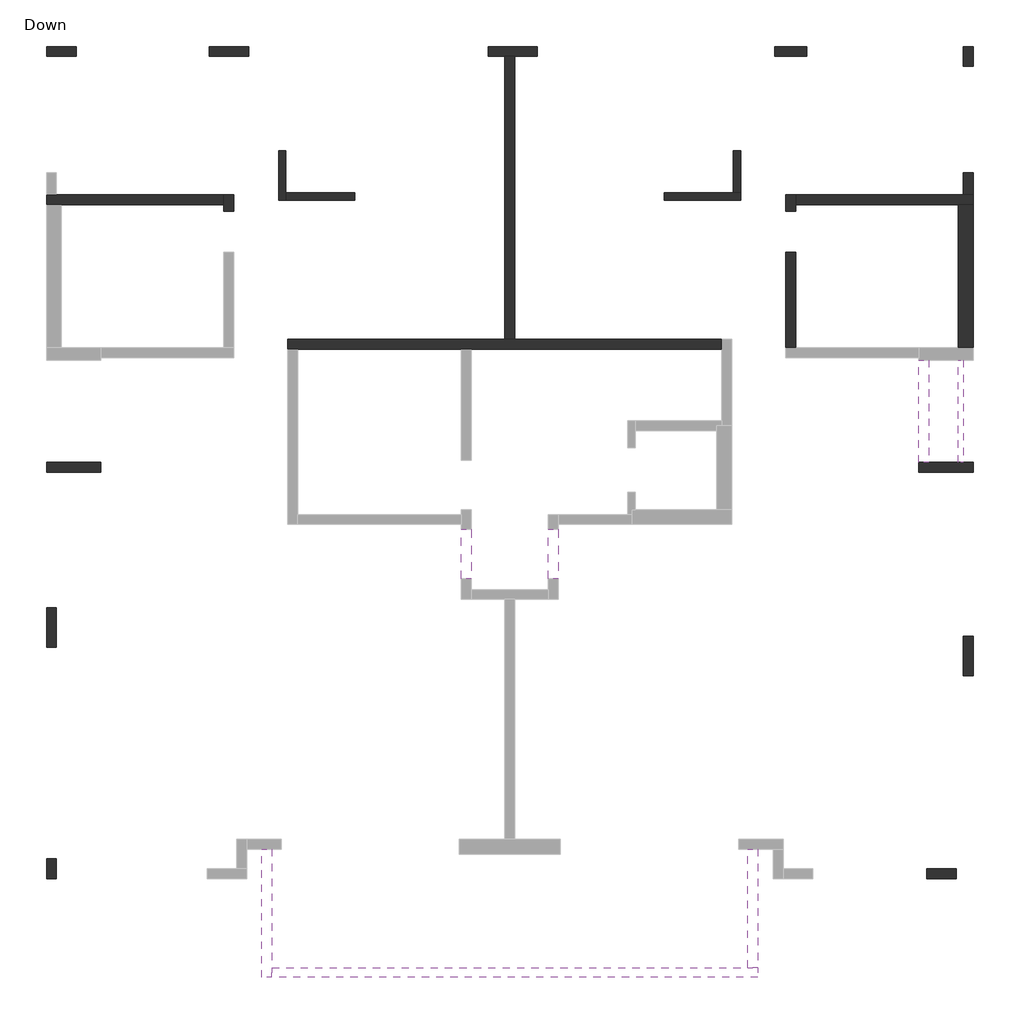
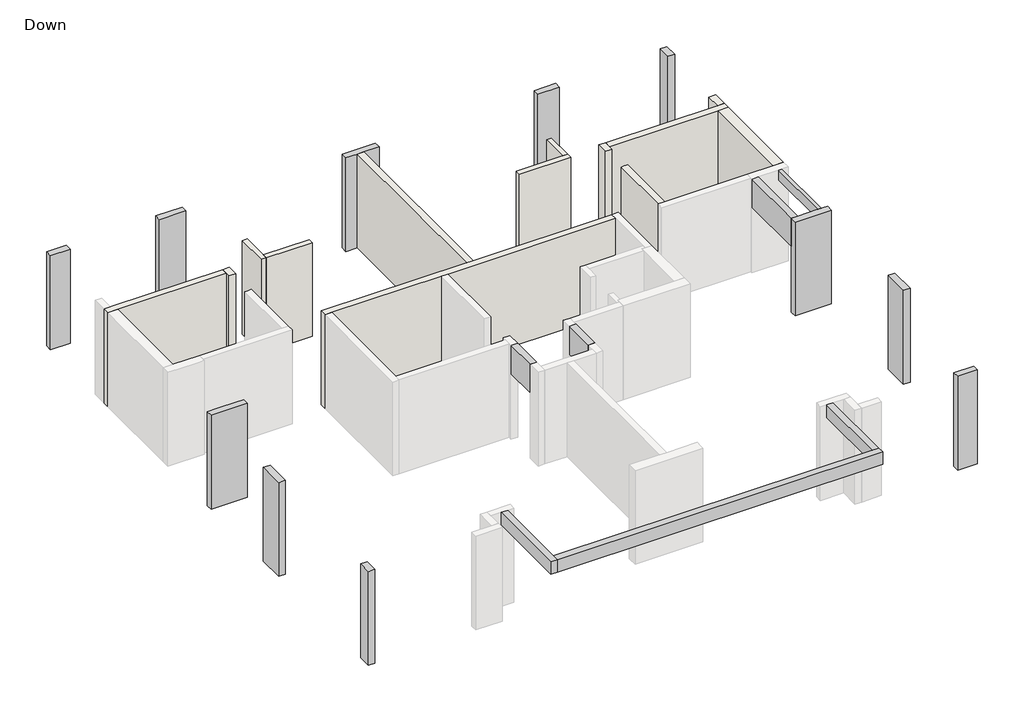
# One storey, part 2 of 2: 13 walls, 11 columns, 7 beams.
"""IFC4 building model written with IfcOpenShell, lengths in millimetres."""

from ifc_helpers import new_model, si_unit, origin, place, context, project, spatial, faceted_brep, element, save

model = new_model("IFC4")

# Units and contexts
model_context = context("Model", 3, world=origin())
ifc_project = project(units=[si_unit("LENGTHUNIT", "METRE", prefix="MILLI")], contexts=[model_context])

# Site, building, storey
site = spatial("IfcSite", under=ifc_project)
building = spatial("IfcBuilding", under=site)
storey = spatial("IfcBuildingStorey", under=building, Name="Down", Elevation=0.0)

# Beams
placement = place(None, origin())
element("IfcBeam", 1, ObjectType="Concrete Rectengular Beam : 10/30", at=placement, inside=storey, context=model_context, shape_type="Brep", body=[
    faceted_brep([(-29340.5251854, 29710.9648817, 3000.0), (-29240.5251854, 29710.9648817, 3000.0), (-29240.5251854, 31780.84273, 3000.0), (-29340.5251854, 31780.84273, 3000.0), (-29240.5251854, 29710.9648817, 2700.0), (-29240.5251854, 31780.84273, 2700.0), (-29340.5251854, 29710.9648817, 2700.0), (-29340.5251854, 31780.84273, 2700.0), (-29340.5251854, 29710.9648817, 2850.0), (-29340.5251854, 31780.84273, 2850.0)], [[[0, 1, 2, 3]], [[1, 4, 5, 2]], [[4, 6, 7, 5]], [[6, 8, 0, 3, 9, 7]], [[1, 0, 8, 6, 4]], [[3, 2, 5, 7, 9]]]),
])
element("IfcBeam", 2, ObjectType="Concrete Rectengular Beam : 20/40", at=placement, inside=storey, context=model_context, shape_type="Brep", body=[
    faceted_brep([(-43443.3137014, 19281.1095176, 3000.0), (-43243.3137014, 19281.1095176, 3000.0), (-43243.3137014, 19481.1095176, 3000.0), (-43243.3137014, 21880.2897882, 3000.0), (-43443.3137014, 21880.2897882, 3000.0), (-43443.3137014, 19281.1095176, 2600.0), (-43443.3137014, 21880.2897882, 2600.0), (-43243.3137014, 19281.1095176, 2600.0), (-43243.3137014, 21880.2897882, 2600.0), (-43243.3137014, 19481.1095176, 2600.0), (-43243.3137014, 21880.2897882, 2800.0)], [[[0, 1, 2, 3, 4]], [[5, 0, 4, 6]], [[7, 5, 6, 8, 9]], [[1, 7, 9, 8, 10, 3, 2]], [[1, 0, 5, 7]], [[4, 3, 10, 8, 6]]]),
])
element("IfcBeam", 3, ObjectType="Concrete Rectengular Beam : 20/40", at=placement, inside=storey, context=model_context, shape_type="Brep", body=[
    faceted_brep([(-33405.0891993, 19281.1095176, 3000.0), (-33405.0891993, 19481.1095176, 3000.0), (-33605.0891993, 19481.1095176, 3000.0), (-43243.3137014, 19481.1095176, 3000.0), (-43243.3137014, 19281.1095176, 3000.0), (-33405.0891993, 19281.1095176, 2600.0), (-43243.3137014, 19281.1095176, 2600.0), (-33405.0891993, 19481.1095176, 2600.0), (-43243.3137014, 19481.1095176, 2600.0), (-33605.0891993, 19481.1095176, 2600.0), (-43243.3137014, 19481.1095176, 2800.0)], [[[0, 1, 2, 3, 4]], [[5, 0, 4, 6]], [[7, 5, 6, 8, 9]], [[1, 7, 9, 8, 10, 3, 2]], [[4, 3, 10, 8, 6]], [[1, 0, 5, 7]]]),
])
element("IfcBeam", 4, ObjectType="Concrete Rectengular Beam : 20/40", at=placement, inside=storey, context=model_context, shape_type="Brep", body=[
    faceted_brep([(-33605.0891993, 19481.1095176, 3000.0), (-33405.0891993, 19481.1095176, 3000.0), (-33405.0891993, 21880.2897882, 3000.0), (-33605.0891993, 21880.2897882, 3000.0), (-33405.0891993, 19481.1095176, 2600.0), (-33405.0891993, 21880.2897882, 2600.0), (-33605.0891993, 19481.1095176, 2600.0), (-33605.0891993, 21880.2897882, 2600.0), (-33605.0891993, 19481.1095176, 2800.0), (-33605.0891993, 21880.2897882, 2800.0)], [[[0, 1, 2, 3]], [[1, 4, 5, 2]], [[4, 6, 7, 5]], [[6, 8, 0, 3, 9, 7]], [[1, 0, 8, 6, 4]], [[3, 2, 5, 7, 9]]]),
])
element("IfcBeam", 5, ObjectType="Concrete Rectengular Beam : 20/90", at=placement, inside=storey, context=model_context, shape_type="Brep", body=[
    faceted_brep([(-37644.7021495, 27352.982888, 3000.0), (-37444.7021495, 27352.982888, 3000.0), (-37444.7021495, 28354.1914622, 3000.0), (-37644.7021495, 28354.1914622, 3000.0), (-37644.7021495, 28354.1914622, 2780.0), (-37644.7021495, 28354.1914622, 2100.0), (-37644.7021495, 27352.982888, 2100.0), (-37644.7021495, 27352.982888, 2780.0), (-37444.7021495, 27352.982888, 2100.0), (-37444.7021495, 28354.1914622, 2100.0), (-37444.7021495, 27352.982888, 2780.0), (-37444.7021495, 28354.1914622, 2780.0)], [[[0, 1, 2, 3]], [[0, 3, 4, 5, 6, 7]], [[8, 6, 5, 9]], [[2, 1, 10, 8, 9, 11]], [[1, 0, 7, 6, 8, 10]], [[3, 2, 11, 9, 5, 4]]]),
])
element("IfcBeam", 6, ObjectType="Concrete Rectengular Beam : 20/90", at=placement, inside=storey, context=model_context, shape_type="Brep", body=[
    faceted_brep([(-39404.7173594, 27352.982888, 3000.0), (-39204.7173594, 27352.982888, 3000.0), (-39204.7173594, 28354.1914622, 3000.0), (-39404.7173594, 28354.1914622, 3000.0), (-39404.7173594, 27352.982888, 2100.0), (-39404.7173594, 27352.982888, 2780.0), (-39404.7173594, 28354.1914622, 2780.0), (-39404.7173594, 28354.1914622, 2100.0), (-39204.7173594, 27352.982888, 2100.0), (-39204.7173594, 28354.1914622, 2100.0), (-39204.7173594, 27352.982888, 2780.0), (-39204.7173594, 28354.1914622, 2780.0)], [[[0, 1, 2, 3]], [[4, 5, 0, 3, 6, 7]], [[8, 4, 7, 9]], [[2, 1, 10, 8, 9, 11]], [[1, 0, 5, 4, 8, 10]], [[3, 2, 11, 9, 7, 6]]]),
])
element("IfcBeam", 7, ObjectType="Concrete Rectengular Beam : 20/90", at=placement, inside=storey, context=model_context, shape_type="Brep", body=[
    faceted_brep([(-30144.302346, 29710.9648817, 3000.0), (-29944.302346, 29710.9648817, 3000.0), (-29944.302346, 31780.84273, 3000.0), (-30144.302346, 31780.84273, 3000.0), (-30144.302346, 31780.84273, 2780.0), (-30144.302346, 31780.84273, 2100.0), (-30144.302346, 29710.9648817, 2100.0), (-30144.302346, 29710.9648817, 2780.0), (-29944.302346, 29710.9648817, 2100.0), (-29944.302346, 31780.84273, 2100.0), (-29944.302346, 29710.9648817, 2850.0), (-29944.302346, 31780.84273, 2850.0)], [[[0, 1, 2, 3]], [[0, 3, 4, 5, 6, 7]], [[8, 6, 5, 9]], [[1, 10, 8, 9, 11, 2]], [[1, 0, 7, 6, 8, 10]], [[3, 2, 11, 9, 5, 4]]]),
])

# Columns
element("IfcColumn", 8, ObjectType="Concrete Rectengular Column : 20/100", at=placement, inside=storey, context=model_context, shape_type="Brep", body=[
    faceted_brep([(-38865.9301848, 38131.0505674, 0.0), (-37865.9301848, 38131.0505674, 0.0), (-37865.9301848, 37931.0505674, 0.0), (-38325.2180585, 37931.0505674, 0.0), (-38525.2180585, 37931.0505674, 0.0), (-38865.9301848, 37931.0505674, 0.0), (-38865.9301848, 38131.0505674, 3000.0), (-37865.9301848, 38131.0505674, 3000.0), (-37865.9301848, 38131.0505674, 2780.0), (-38865.9301848, 38131.0505674, 2780.0), (-37865.9301848, 37931.0505674, 3000.0), (-37865.9301848, 37931.0505674, 2780.0), (-38325.2180585, 37931.0505674, 3000.0), (-38525.2180585, 37931.0505674, 3000.0), (-38865.9301848, 37931.0505674, 3000.0), (-38865.9301848, 37931.0505674, 2780.0)], [[[0, 1, 2, 3, 4, 5]], [[6, 7, 8, 1, 0, 9]], [[7, 10, 11, 2, 1, 8]], [[10, 12, 13, 14, 15, 5, 4, 3, 2, 11]], [[14, 6, 9, 0, 5, 15]], [[6, 14, 13, 12, 10, 7]]]),
])
element("IfcColumn", 9, ObjectType="Concrete Rectengular Column : 20/110", at=placement, inside=storey, context=model_context, shape_type="Brep", body=[
    faceted_brep([(-47805.7952795, 29710.9648817, 0.0), (-46705.7952795, 29710.9648817, 0.0), (-46705.7952795, 29510.9648817, 0.0), (-47805.7952795, 29510.9648817, 0.0), (-47805.7952795, 29710.9648817, 3000.0), (-47505.2156022, 29710.9648817, 3000.0), (-46905.7952795, 29710.9648817, 3000.0), (-46705.7952795, 29710.9648817, 3000.0), (-46705.7952795, 29510.9648817, 3000.0), (-46705.7952795, 29510.9648817, 2780.0), (-47805.7952795, 29510.9648817, 3000.0), (-47805.7952795, 29510.9648817, 2780.0)], [[[0, 1, 2, 3]], [[4, 5, 6, 7, 1, 0]], [[7, 8, 9, 2, 1]], [[8, 10, 11, 3, 2, 9]], [[10, 4, 0, 3, 11]], [[4, 10, 8, 7, 6, 5]]]),
])
element("IfcColumn", 10, ObjectType="Concrete Rectengular Column : 20/110", at=placement, inside=storey, context=model_context, shape_type="Brep", body=[
    faceted_brep([(-30144.302346, 29710.9648817, 0.0), (-29044.302346, 29710.9648817, 0.0), (-29044.302346, 29510.9648817, 0.0), (-30144.302346, 29510.9648817, 0.0), (-30144.302346, 29710.9648817, 3000.0), (-29944.302346, 29710.9648817, 3000.0), (-29340.5251854, 29710.9648817, 3000.0), (-29044.302346, 29710.9648817, 3000.0), (-29044.302346, 29510.9648817, 3000.0), (-29045.7952795, 29510.9648817, 3000.0), (-30144.302346, 29510.9648817, 3000.0), (-30144.302346, 29510.9648817, 2780.0)], [[[0, 1, 2, 3]], [[4, 5, 6, 7, 1, 0]], [[7, 8, 2, 1]], [[8, 9, 10, 11, 3, 2]], [[10, 4, 0, 3, 11]], [[4, 10, 9, 8, 7, 6, 5]]]),
])
element("IfcColumn", 11, ObjectType="Concrete Rectengular Column : 20/40", at=placement, inside=storey, context=model_context, shape_type="Brep", body=[
    faceted_brep([(-29244.7343642, 37731.0505674, 0.0), (-29244.7343642, 38131.0505674, 0.0), (-29044.7343642, 38131.0505674, 0.0), (-29044.7343642, 37731.0505674, 0.0), (-29244.7343642, 37731.0505674, 3000.0), (-29244.7343642, 38131.0505674, 3000.0), (-29244.7343642, 38131.0505674, 2780.0), (-29244.7343642, 37731.0505674, 2780.0), (-29044.7343642, 38131.0505674, 3000.0), (-29044.7343642, 37731.0505674, 3000.0), (-29044.7343642, 37731.0505674, 2780.0)], [[[0, 1, 2, 3]], [[4, 5, 6, 1, 0, 7]], [[5, 8, 2, 1, 6]], [[8, 9, 10, 3, 2]], [[9, 4, 7, 0, 3, 10]], [[4, 9, 8, 5]]]),
])
element("IfcColumn", 12, ObjectType="Concrete Rectengular Column : 20/40", at=placement, inside=storey, context=model_context, shape_type="Brep", body=[
    faceted_brep([(-47605.7952795, 21680.2897882, 0.0), (-47605.7952795, 21280.2897882, 0.0), (-47805.7952795, 21280.2897882, 0.0), (-47805.7952795, 21680.2897882, 0.0), (-47605.7952795, 21680.2897882, 3000.0), (-47605.7952795, 21280.2897882, 3000.0), (-47605.7952795, 21280.2897882, 2780.0), (-47605.7952795, 21680.2897882, 2780.0), (-47805.7952795, 21280.2897882, 3000.0), (-47805.7952795, 21680.2897882, 3000.0), (-47805.7952795, 21680.2897882, 2780.0)], [[[0, 1, 2, 3]], [[4, 5, 6, 1, 0, 7]], [[5, 8, 2, 1, 6]], [[8, 9, 10, 3, 2]], [[9, 4, 7, 0, 3, 10]], [[4, 9, 8, 5]]]),
])
element("IfcColumn", 13, ObjectType="Concrete Rectengular Column : 20/60", at=placement, inside=storey, context=model_context, shape_type="Brep", body=[
    faceted_brep([(-47805.7952795, 38131.0505674, 0.0), (-47205.7952795, 38131.0505674, 0.0), (-47205.7952795, 37931.0505674, 0.0), (-47805.7952795, 37931.0505674, 0.0), (-47805.7952795, 38131.0505674, 3000.0), (-47205.7952795, 38131.0505674, 3000.0), (-47205.7952795, 38131.0505674, 2780.0), (-47205.7952795, 37931.0505674, 3000.0), (-47205.7952795, 37931.0505674, 2780.0), (-47805.7952795, 37931.0505674, 3000.0)], [[[0, 1, 2, 3]], [[4, 5, 6, 1, 0]], [[5, 7, 8, 2, 1, 6]], [[7, 9, 3, 2, 8]], [[9, 4, 0, 3]], [[4, 9, 7, 5]]]),
])
element("IfcColumn", 14, ObjectType="Concrete Rectengular Column : 20/60", at=placement, inside=storey, context=model_context, shape_type="Brep", body=[
    faceted_brep([(-29982.308052, 21480.2897882, 0.0), (-29382.308052, 21480.2897882, 0.0), (-29382.308052, 21280.2897882, 0.0), (-29982.308052, 21280.2897882, 0.0), (-29982.308052, 21480.2897882, 3000.0), (-29382.308052, 21480.2897882, 3000.0), (-29382.308052, 21480.2897882, 2780.0), (-29982.308052, 21480.2897882, 2780.0), (-29382.308052, 21280.2897882, 3000.0), (-29382.308052, 21280.2897882, 2780.0), (-29982.308052, 21280.2897882, 3000.0), (-29982.308052, 21280.2897882, 2780.0)], [[[0, 1, 2, 3]], [[4, 5, 6, 1, 0, 7]], [[5, 8, 9, 2, 1, 6]], [[8, 10, 11, 3, 2, 9]], [[10, 4, 7, 0, 3, 11]], [[4, 10, 8, 5]]]),
])
element("IfcColumn", 15, ObjectType="Concrete Rectengular Column : 20/65", at=placement, inside=storey, context=model_context, shape_type="Brep", body=[
    faceted_brep([(-33061.2774622, 38131.0505674, 0.0), (-32411.2774622, 38131.0505674, 0.0), (-32411.2774622, 37931.0505674, 0.0), (-33061.2774622, 37931.0505674, 0.0), (-33061.2774622, 38131.0505674, 3000.0), (-32411.2774622, 38131.0505674, 3000.0), (-32411.2774622, 38131.0505674, 2780.0), (-33061.2774622, 38131.0505674, 2780.0), (-32411.2774622, 37931.0505674, 3000.0), (-32411.2774622, 37931.0505674, 2780.0), (-33061.2774622, 37931.0505674, 3000.0), (-33061.2774622, 37931.0505674, 2780.0)], [[[0, 1, 2, 3]], [[4, 5, 6, 1, 0, 7]], [[5, 8, 9, 2, 1, 6]], [[8, 10, 11, 3, 2, 9]], [[10, 4, 7, 0, 3, 11]], [[4, 10, 8, 5]]]),
])
element("IfcColumn", 16, ObjectType="Concrete Rectengular Column : 20/80", at=placement, inside=storey, context=model_context, shape_type="Brep", body=[
    faceted_brep([(-44508.0144156, 38131.0505674, 0.0), (-43708.0144156, 38131.0505674, 0.0), (-43708.0144156, 37931.0505674, 0.0), (-44508.0144156, 37931.0505674, 0.0), (-44508.0144156, 38131.0505674, 3000.0), (-43708.0144156, 38131.0505674, 3000.0), (-43708.0144156, 38131.0505674, 2780.0), (-44508.0144156, 38131.0505674, 2780.0), (-43708.0144156, 37931.0505674, 3000.0), (-43708.0144156, 37931.0505674, 2780.0), (-44508.0144156, 37931.0505674, 3000.0), (-44508.0144156, 37931.0505674, 2780.0)], [[[0, 1, 2, 3]], [[4, 5, 6, 1, 0, 7]], [[5, 8, 9, 2, 1, 6]], [[8, 10, 11, 3, 2, 9]], [[10, 4, 7, 0, 3, 11]], [[4, 10, 8, 5]]]),
])
element("IfcColumn", 17, ObjectType="Concrete Rectengular Column : 20/80", at=placement, inside=storey, context=model_context, shape_type="Brep", body=[
    faceted_brep([(-47605.7952795, 26768.694731, 0.0), (-47605.7952795, 25968.694731, 0.0), (-47805.7952795, 25968.694731, 0.0), (-47805.7952795, 26768.694731, 0.0), (-47605.7952795, 26768.694731, 3000.0), (-47605.7952795, 25968.694731, 3000.0), (-47605.7952795, 25968.694731, 2780.0), (-47605.7952795, 26768.694731, 2780.0), (-47805.7952795, 25968.694731, 3000.0), (-47805.7952795, 25968.694731, 2780.0), (-47805.7952795, 26768.694731, 3000.0), (-47805.7952795, 26768.694731, 2780.0)], [[[0, 1, 2, 3]], [[4, 5, 6, 1, 0, 7]], [[5, 8, 9, 2, 1, 6]], [[8, 10, 11, 3, 2, 9]], [[10, 4, 7, 0, 3, 11]], [[4, 10, 8, 5]]]),
])
element("IfcColumn", 18, ObjectType="Concrete Rectengular Column : 20/80", at=placement, inside=storey, context=model_context, shape_type="Brep", body=[
    faceted_brep([(-29045.7952795, 26190.9393744, 0.0), (-29045.7952795, 25390.9393744, 0.0), (-29245.7952795, 25390.9393744, 0.0), (-29245.7952795, 26190.9393744, 0.0), (-29045.7952795, 26190.9393744, 3000.0), (-29045.7952795, 25390.9393744, 3000.0), (-29045.7952795, 25390.9393744, 2780.0), (-29045.7952795, 26190.9393744, 2780.0), (-29245.7952795, 25390.9393744, 3000.0), (-29245.7952795, 25390.9393744, 2780.0), (-29245.7952795, 26190.9393744, 3000.0), (-29245.7952795, 26190.9393744, 2780.0)], [[[0, 1, 2, 3]], [[4, 5, 6, 1, 0, 7]], [[5, 8, 9, 2, 1, 6]], [[8, 10, 11, 3, 2, 9]], [[10, 4, 7, 0, 3, 11]], [[4, 10, 8, 5]]]),
])

# Walls
element("IfcWall", 19, ObjectType="15", at=placement, inside=storey, context=model_context, shape_type="Brep", body=[
    faceted_brep([(-43108.8833647, 36022.8722618, 0.0), (-43108.8833647, 35023.7904306, 0.0), (-43108.8833647, 35023.7904306, 2780.0), (-43108.8833647, 35023.7904306, 3000.0), (-43108.8833647, 36022.8722618, 3000.0), (-43108.8833647, 36022.8722618, 2780.0), (-42958.8833647, 36022.8722618, 0.0), (-42958.8833647, 36022.8722618, 2780.0), (-42958.8833647, 36022.8722618, 3000.0), (-42958.8833647, 35173.7904306, 3000.0), (-42958.8833647, 35023.7904306, 3000.0), (-42958.8833647, 35023.7904306, 0.0), (-42958.8833647, 35173.7904306, 0.0)], [[[0, 1, 2, 3, 4, 5]], [[6, 7, 8, 9, 10, 11, 12]], [[1, 0, 6, 12, 11]], [[4, 3, 10, 9, 8]], [[0, 5, 4, 8, 7, 6]], [[3, 2, 1, 11, 10]]]),
])
element("IfcWall", 20, ObjectType="15", at=placement, inside=storey, context=model_context, shape_type="Brep", body=[
    faceted_brep([(-42958.8833647, 35023.7904306, 0.0), (-41563.7602683, 35023.7904306, 0.0), (-41563.7602683, 35023.7904306, 2780.0), (-41563.7602683, 35023.7904306, 3000.0), (-42958.8833647, 35023.7904306, 3000.0), (-42958.8833647, 35173.7904306, 0.0), (-42958.8833647, 35173.7904306, 2780.0), (-42958.8833647, 35173.7904306, 3000.0), (-41563.7602683, 35173.7904306, 3000.0), (-41563.7602683, 35173.7904306, 2780.0), (-41563.7602683, 35173.7904306, 0.0)], [[[0, 1, 2, 3, 4]], [[5, 6, 7, 8, 9, 10]], [[1, 0, 5, 10]], [[3, 2, 1, 10, 9, 8]], [[4, 3, 8, 7]], [[0, 4, 7, 6, 5]]]),
])
element("IfcWall", 21, ObjectType="15", at=placement, inside=storey, context=model_context, shape_type="Brep", body=[
    faceted_brep([(-35302.6288773, 35023.7904306, 0.0), (-33753.2522949, 35023.7904306, 0.0), (-33753.2522949, 35023.7904306, 2780.0), (-33753.2522949, 35023.7904306, 3000.0), (-35302.6288773, 35023.7904306, 3000.0), (-35302.6288773, 35023.7904306, 2780.0), (-35302.6288773, 35173.7904306, 0.0), (-35302.6288773, 35173.7904306, 2780.0), (-35302.6288773, 35173.7904306, 3000.0), (-33903.2522949, 35173.7904306, 3000.0), (-33753.2522949, 35173.7904306, 3000.0), (-33753.2522949, 35173.7904306, 0.0), (-33903.2522949, 35173.7904306, 0.0)], [[[0, 1, 2, 3, 4, 5]], [[6, 7, 8, 9, 10, 11, 12]], [[1, 0, 6, 12, 11]], [[4, 3, 10, 9, 8]], [[0, 5, 4, 8, 7, 6]], [[3, 2, 1, 11, 10]]]),
])
element("IfcWall", 22, ObjectType="15", at=placement, inside=storey, context=model_context, shape_type="Brep", body=[
    faceted_brep([(-33753.2522949, 35173.7904306, 0.0), (-33753.2522949, 36022.8722618, 0.0), (-33753.2522949, 36022.8722618, 2780.0), (-33753.2522949, 36022.8722618, 3000.0), (-33753.2522949, 35173.7904306, 3000.0), (-33903.2522949, 35173.7904306, 0.0), (-33903.2522949, 35173.7904306, 2780.0), (-33903.2522949, 35173.7904306, 3000.0), (-33903.2522949, 36022.8722618, 3000.0), (-33903.2522949, 36022.8722618, 2780.0), (-33903.2522949, 36022.8722618, 0.0)], [[[0, 1, 2, 3, 4]], [[5, 6, 7, 8, 9, 10]], [[1, 0, 5, 10]], [[3, 2, 1, 10, 9, 8]], [[4, 3, 8, 7]], [[0, 4, 7, 6, 5]]]),
])
element("IfcWall", 23, ObjectType="20", at=placement, inside=storey, context=model_context, shape_type="Brep", body=[
    faceted_brep([(-34133.139307, 32204.3938202, 0.0), (-38325.2180585, 32204.3938202, 0.0), (-38525.2180585, 32204.3938202, 0.0), (-42920.5336878, 32204.3938202, 0.0), (-42920.5336878, 32204.3938202, 2780.0), (-42920.5336878, 32204.3938202, 3000.0), (-38525.2180585, 32204.3938202, 3000.0), (-38325.2180585, 32204.3938202, 3000.0), (-34133.139307, 32204.3938202, 3000.0), (-34133.139307, 32004.3938202, 0.0), (-34133.139307, 32004.3938202, 2780.0), (-34133.139307, 32004.3938202, 3000.0), (-39204.7173594, 32004.3938202, 3000.0), (-39404.7173594, 32004.3938202, 3000.0), (-42720.5336878, 32004.3938202, 3000.0), (-42920.5336878, 32004.3938202, 3000.0), (-42920.5336878, 32004.3938202, 0.0), (-42720.5336878, 32004.3938202, 0.0), (-39404.7173594, 32004.3938202, 0.0), (-39204.7173594, 32004.3938202, 0.0)], [[[0, 1, 2, 3, 4, 5, 6, 7, 8]], [[9, 10, 11, 12, 13, 14, 15, 16, 17, 18, 19]], [[3, 2, 1, 0, 9, 19, 18, 17, 16]], [[8, 7, 6, 5, 15, 14, 13, 12, 11]], [[0, 8, 11, 10, 9]], [[5, 4, 3, 16, 15]]]),
])
element("IfcWall", 24, ObjectType="20", at=placement, inside=storey, context=model_context, shape_type="Brep", body=[
    faceted_brep([(-38325.2180585, 32204.3938202, 0.0), (-38325.2180585, 37931.0505674, 0.0), (-38325.2180585, 37931.0505674, 2780.0), (-38325.2180585, 37931.0505674, 3000.0), (-38325.2180585, 32204.3938202, 3000.0), (-38325.2180585, 32204.3938202, 2780.0), (-38525.2180585, 32204.3938202, 0.0), (-38525.2180585, 32204.3938202, 2780.0), (-38525.2180585, 32204.3938202, 3000.0), (-38525.2180585, 37931.0505674, 3000.0), (-38525.2180585, 37931.0505674, 2780.0), (-38525.2180585, 37931.0505674, 0.0)], [[[0, 1, 2, 3, 4, 5]], [[6, 7, 8, 9, 10, 11]], [[1, 0, 6, 11]], [[3, 2, 1, 11, 10, 9]], [[4, 3, 9, 8]], [[0, 5, 4, 8, 7, 6]]]),
])
element("IfcWall", 25, ObjectType="20", at=placement, inside=storey, context=model_context, shape_type="Brep", body=[
    faceted_brep([(-29244.7343642, 35580.4654108, 0.0), (-29244.7343642, 35129.640202, 0.0), (-29244.7343642, 35129.640202, 2780.0), (-29244.7343642, 35129.640202, 3000.0), (-29244.7343642, 35580.4654108, 3000.0), (-29244.7343642, 35580.4654108, 2780.0), (-29044.7343642, 35580.4654108, 0.0), (-29044.7343642, 35580.4654108, 2780.0), (-29044.7343642, 35580.4654108, 3000.0), (-29044.7343642, 35129.640202, 3000.0), (-29044.7343642, 35129.640202, 0.0)], [[[0, 1, 2, 3, 4, 5]], [[6, 7, 8, 9, 10]], [[1, 0, 6, 10]], [[4, 3, 9, 8]], [[0, 5, 4, 8, 7, 6]], [[3, 2, 1, 10, 9]]]),
])
element("IfcWall", 26, ObjectType="20", at=placement, inside=storey, context=model_context, shape_type="Brep", body=[
    faceted_brep([(-32634.5879334, 32030.84273, 0.0), (-32634.5879334, 33965.4699454, 0.0), (-32634.5879334, 33965.4699454, 2780.0), (-32634.5879334, 33965.4699454, 3000.0), (-32634.5879334, 32030.84273, 3000.0), (-32634.5879334, 32030.84273, 2780.0), (-32834.5879334, 32030.84273, 0.0), (-32834.5879334, 32030.84273, 3000.0), (-32834.5879334, 33965.4699454, 3000.0), (-32834.5879334, 33965.4699454, 2780.0), (-32834.5879334, 33965.4699454, 0.0), (-32734.5879334, 33965.4699454, 3000.0)], [[[0, 1, 2, 3, 4, 5]], [[6, 7, 8, 9, 10]], [[1, 0, 6, 10]], [[3, 2, 1, 10, 9, 8, 11]], [[4, 3, 11, 8, 7]], [[0, 5, 4, 7, 6]]]),
])
element("IfcWall", 27, ObjectType="20", at=placement, inside=storey, context=model_context, shape_type="Brep", body=[
    faceted_brep([(-32634.5879334, 34793.0831223, 0.0), (-32634.5879334, 34929.640202, 0.0), (-32634.5879334, 35129.640202, 0.0), (-32634.5879334, 35129.640202, 3000.0), (-32634.5879334, 34929.640202, 3000.0), (-32634.5879334, 34793.0831223, 3000.0), (-32634.5879334, 34793.0831223, 2780.0), (-32834.5879334, 34793.0831223, 0.0), (-32834.5879334, 34793.0831223, 2780.0), (-32834.5879334, 34793.0831223, 3000.0), (-32834.5879334, 35129.640202, 3000.0), (-32834.5879334, 35129.640202, 2780.0), (-32834.5879334, 35129.640202, 0.0), (-32734.5879334, 34793.0831223, 3000.0)], [[[0, 1, 2, 3, 4, 5, 6]], [[7, 8, 9, 10, 11, 12]], [[2, 1, 0, 7, 12]], [[5, 4, 3, 10, 9, 13]], [[0, 6, 5, 13, 9, 8, 7]], [[3, 2, 12, 11, 10]]]),
])
element("IfcWall", 28, ObjectType="20", at=placement, inside=storey, context=model_context, shape_type="Brep", body=[
    faceted_brep([(-32634.5879334, 34929.640202, 0.0), (-29344.7343642, 34929.640202, 0.0), (-29044.7343642, 34929.640202, 0.0), (-29044.7343642, 34929.640202, 3000.0), (-29344.7343642, 34929.640202, 3000.0), (-32634.5879334, 34929.640202, 3000.0), (-32634.5879334, 34929.640202, 2780.0), (-32634.5879334, 35129.640202, 0.0), (-32634.5879334, 35129.640202, 3000.0), (-29244.7343642, 35129.640202, 3000.0), (-29044.7343642, 35129.640202, 3000.0), (-29044.7343642, 35129.640202, 0.0), (-29244.7343642, 35129.640202, 0.0)], [[[0, 1, 2, 3, 4, 5, 6]], [[7, 8, 9, 10, 11, 12]], [[2, 1, 0, 7, 12, 11]], [[5, 4, 3, 10, 9, 8]], [[0, 6, 5, 8, 7]], [[3, 2, 11, 10]]]),
])
element("IfcWall", 29, ObjectType="20", at=placement, inside=storey, context=model_context, shape_type="Brep", body=[
    faceted_brep([(-44015.8481835, 34793.0831223, 0.0), (-44015.8481835, 35129.640202, 0.0), (-44015.8481835, 35129.640202, 2780.0), (-44015.8481835, 35129.640202, 3000.0), (-44015.8481835, 34793.0831223, 3000.0), (-44015.8481835, 34793.0831223, 2780.0), (-44215.8481835, 34793.0831223, 0.0), (-44215.8481835, 34793.0831223, 2780.0), (-44215.8481835, 34793.0831223, 3000.0), (-44215.8481835, 34929.640202, 3000.0), (-44215.8481835, 35129.640202, 3000.0), (-44215.8481835, 35129.640202, 0.0), (-44215.8481835, 34929.640202, 0.0), (-44113.8149674, 34793.0831223, 3000.0)], [[[0, 1, 2, 3, 4, 5]], [[6, 7, 8, 9, 10, 11, 12]], [[1, 0, 6, 12, 11]], [[4, 3, 10, 9, 8, 13]], [[0, 5, 4, 13, 8, 7, 6]], [[3, 2, 1, 11, 10]]]),
])
element("IfcWall", 30, ObjectType="20", at=placement, inside=storey, context=model_context, shape_type="Brep", body=[
    faceted_brep([(-44215.8481835, 35129.640202, 0.0), (-47605.7017527, 35129.640202, 0.0), (-47805.7017527, 35129.640202, 0.0), (-47805.7017527, 35129.640202, 3000.0), (-47605.7017527, 35129.640202, 3000.0), (-44215.8481835, 35129.640202, 3000.0), (-44215.8481835, 34929.640202, 0.0), (-44215.8481835, 34929.640202, 2780.0), (-44215.8481835, 34929.640202, 3000.0), (-47505.7017527, 34929.640202, 3000.0), (-47805.7017527, 34929.640202, 3000.0), (-47805.7017527, 34929.640202, 0.0), (-47505.7017527, 34929.640202, 0.0)], [[[0, 1, 2, 3, 4, 5]], [[6, 7, 8, 9, 10, 11, 12]], [[2, 1, 0, 6, 12, 11]], [[5, 4, 3, 10, 9, 8]], [[0, 5, 8, 7, 6]], [[3, 2, 11, 10]]]),
])
element("IfcWall", 31, ObjectType="30", at=placement, inside=storey, context=model_context, shape_type="Brep", body=[
    faceted_brep([(-29344.7343642, 34929.640202, 0.0), (-29344.7343642, 32030.84273, 0.0), (-29344.7343642, 32030.84273, 2780.0), (-29344.7343642, 32030.84273, 3000.0), (-29344.7343642, 34929.640202, 3000.0), (-29344.7343642, 34929.640202, 2780.0), (-29044.7343642, 34929.640202, 0.0), (-29044.7343642, 34929.640202, 3000.0), (-29044.7343642, 32030.84273, 3000.0), (-29044.7343642, 32030.84273, 0.0)], [[[0, 1, 2, 3, 4, 5]], [[6, 7, 8, 9]], [[1, 0, 6, 9]], [[4, 3, 8, 7]], [[3, 2, 1, 9, 8]], [[0, 5, 4, 7, 6]]]),
])

save(model, "model.ifc")

# Revit data of these elements
# Type "Concrete Rectengular Beam : 10/30"
#   Length [instance default] = 152.4 cm
#   b = 10 cm
#   h = 30 cm
#   Structural Material [instance default] = Concrete
#   Assembly Code = ""
# Type "Concrete Rectengular Beam : 20/40"
#   Keynote = "09000"
#   Length [instance default] = 152.4 cm
#   b = 20 cm
#   h = 40 cm
#   Structural Material [instance default] = Concrete
#   Assembly Code = ""
# Type "Concrete Rectengular Beam : 20/90"
#   Length [instance default] = 152.4 cm
#   b = 20 cm
#   h = 90 cm
#   Structural Material [instance default] = Concrete
#   Assembly Code = ""
# Type "Concrete Rectengular Column : 20/100"
#   b = 20 cm
#   h = 100 cm
#   Structural Material [instance default] = Concrete
# Type "Concrete Rectengular Column : 20/110"
#   b = 20 cm
#   h = 110 cm
#   Structural Material [instance default] = Concrete
# Type "Concrete Rectengular Column : 20/40"
#   b = 20 cm
#   h = 40 cm
#   Structural Material [instance default] = Concrete
# Type "Concrete Rectengular Column : 20/60"
#   b = 20 cm
#   h = 60 cm
#   Structural Material [instance default] = Concrete
# Type "Concrete Rectengular Column : 20/65"
#   b = 20 cm
#   h = 65 cm
#   Structural Material [instance default] = Concrete
# Type "Concrete Rectengular Column : 20/80"
#   b = 20 cm
#   h = 80 cm
#   Structural Material [instance default] = Concrete
# Type "15"
#   Layers, outside or top first: 15 cm "Concrete" (function 1)
# Type "20"
#   Layers, outside or top first: 20 cm "Concrete" (function 1)
# Type "30"
#   Layers, outside or top first: 30 cm "Concrete" (function 1)
# Element 1 (IfcBeam, "Concrete Rectengular Beam : 10/30")
#   Comments = ""
#   Mark = "B1"
#   SOFiSTiK_AMG_Comments = "Too Narrow Beam /"
#   SOFiSTiK_AMG_Scheduled = yes
#   SOFiSTiK_AMG_Adjusted = yes
#   Structural Material = Concrete
#   Phase Created = New Construction
#   Materials on its faces: "Concrete"
# Element 2 (IfcBeam, "Concrete Rectengular Beam : 20/40")
#   Comments = ""
#   Mark = "B3"
#   SOFiSTiK_AMG_Comments = ""
#   SOFiSTiK_AMG_Scheduled = yes
#   SOFiSTiK_AMG_Adjusted = yes
#   Structural Material = Concrete
#   Phase Created = New Construction
#   Materials on its faces: "Concrete"
# Element 3 (IfcBeam, "Concrete Rectengular Beam : 20/40")
#   Comments = ""
#   Mark = "B4"
#   SOFiSTiK_AMG_Comments = ""
#   SOFiSTiK_AMG_Scheduled = yes
#   SOFiSTiK_AMG_Adjusted = yes
#   Structural Material = Concrete
#   Phase Created = New Construction
#   Materials on its faces: "Concrete"
# Element 4 (IfcBeam, "Concrete Rectengular Beam : 20/40")
#   Comments = ""
#   Mark = "B5"
#   SOFiSTiK_AMG_Comments = ""
#   SOFiSTiK_AMG_Scheduled = yes
#   SOFiSTiK_AMG_Adjusted = yes
#   Structural Material = Concrete
#   Phase Created = New Construction
#   Materials on its faces: "Concrete"
# Element 5 (IfcBeam, "Concrete Rectengular Beam : 20/90")
#   Comments = ""
#   Mark = "B7"
#   SOFiSTiK_AMG_Comments = ""
#   SOFiSTiK_AMG_Scheduled = yes
#   SOFiSTiK_AMG_Adjusted = yes
#   Structural Material = Concrete
#   Phase Created = New Construction
#   Materials on its faces: "Concrete"
# Element 6 (IfcBeam, "Concrete Rectengular Beam : 20/90")
#   Comments = ""
#   Mark = "B8"
#   SOFiSTiK_AMG_Comments = ""
#   SOFiSTiK_AMG_Scheduled = yes
#   SOFiSTiK_AMG_Adjusted = yes
#   Structural Material = Concrete
#   Phase Created = New Construction
#   Materials on its faces: "Concrete"
# Element 7 (IfcBeam, "Concrete Rectengular Beam : 20/90")
#   Comments = ""
#   Mark = "B9"
#   SOFiSTiK_AMG_Comments = ""
#   SOFiSTiK_AMG_Scheduled = yes
#   SOFiSTiK_AMG_Adjusted = yes
#   Structural Material = Concrete
#   Phase Created = New Construction
#   Materials on its faces: "Concrete"
# Element 8 (IfcColumn, "Concrete Rectengular Column : 20/100")
#   Comments = ""
#   Mark = "C1"
#   SOFiSTiK_AMG_Comments = ""
#   SOFiSTiK_AMG_Scheduled = yes
#   SOFiSTiK_AMG_Adjusted = yes
#   Structural Material = Concrete
#   Phase Created = New Construction
#   Materials on its faces: "Concrete"
# Element 9 (IfcColumn, "Concrete Rectengular Column : 20/110")
#   Comments = ""
#   Mark = "C2"
#   SOFiSTiK_AMG_Comments = ""
#   SOFiSTiK_AMG_Scheduled = yes
#   SOFiSTiK_AMG_Adjusted = yes
#   Structural Material = Concrete
#   Phase Created = New Construction
#   Materials on its faces: "Concrete"
# Element 10 (IfcColumn, "Concrete Rectengular Column : 20/110")
#   Comments = ""
#   Mark = "C3"
#   SOFiSTiK_AMG_Comments = ""
#   SOFiSTiK_AMG_Scheduled = yes
#   SOFiSTiK_AMG_Adjusted = yes
#   Structural Material = Concrete
#   Phase Created = New Construction
#   Materials on its faces: "Concrete"
# Element 11 (IfcColumn, "Concrete Rectengular Column : 20/40")
#   Comments = ""
#   Mark = "C6"
#   SOFiSTiK_AMG_Comments = ""
#   SOFiSTiK_AMG_Scheduled = yes
#   SOFiSTiK_AMG_Adjusted = yes
#   Structural Material = Concrete
#   Phase Created = New Construction
#   Materials on its faces: "Concrete"
# Element 12 (IfcColumn, "Concrete Rectengular Column : 20/40")
#   Comments = ""
#   Mark = "C7"
#   SOFiSTiK_AMG_Comments = ""
#   SOFiSTiK_AMG_Scheduled = yes
#   SOFiSTiK_AMG_Adjusted = yes
#   Structural Material = Concrete
#   Phase Created = New Construction
#   Materials on its faces: "Concrete"
# Element 13 (IfcColumn, "Concrete Rectengular Column : 20/60")
#   Comments = ""
#   Mark = "C8"
#   SOFiSTiK_AMG_Comments = ""
#   SOFiSTiK_AMG_Scheduled = yes
#   SOFiSTiK_AMG_Adjusted = yes
#   Structural Material = Concrete
#   Phase Created = New Construction
#   Materials on its faces: "Concrete"
# Element 14 (IfcColumn, "Concrete Rectengular Column : 20/60")
#   Comments = ""
#   Mark = "C9"
#   SOFiSTiK_AMG_Comments = ""
#   SOFiSTiK_AMG_Scheduled = yes
#   SOFiSTiK_AMG_Adjusted = yes
#   Structural Material = Concrete
#   Phase Created = New Construction
#   Materials on its faces: "Concrete"
# Element 15 (IfcColumn, "Concrete Rectengular Column : 20/65")
#   Comments = ""
#   Mark = "C10"
#   SOFiSTiK_AMG_Comments = ""
#   SOFiSTiK_AMG_Scheduled = yes
#   SOFiSTiK_AMG_Adjusted = yes
#   Structural Material = Concrete
#   Phase Created = New Construction
#   Materials on its faces: "Concrete"
# Element 16 (IfcColumn, "Concrete Rectengular Column : 20/80")
#   Comments = ""
#   Mark = "C11"
#   SOFiSTiK_AMG_Comments = ""
#   SOFiSTiK_AMG_Scheduled = yes
#   SOFiSTiK_AMG_Adjusted = yes
#   Structural Material = Concrete
#   Phase Created = New Construction
#   Materials on its faces: "Concrete"
# Element 17 (IfcColumn, "Concrete Rectengular Column : 20/80")
#   Comments = ""
#   Mark = "C12"
#   SOFiSTiK_AMG_Comments = ""
#   SOFiSTiK_AMG_Scheduled = yes
#   SOFiSTiK_AMG_Adjusted = yes
#   Structural Material = Concrete
#   Phase Created = New Construction
#   Materials on its faces: "Concrete"
# Element 18 (IfcColumn, "Concrete Rectengular Column : 20/80")
#   Comments = ""
#   Mark = "C13"
#   SOFiSTiK_AMG_Comments = ""
#   SOFiSTiK_AMG_Scheduled = yes
#   SOFiSTiK_AMG_Adjusted = yes
#   Structural Material = Concrete
#   Phase Created = New Construction
#   Materials on its faces: "Concrete"
# Element 19 (IfcWall, "15")
#   Comments = ""
#   Mark = "W1"
#   SOFiSTiK_EdgeZones = "W1"
#   SOFiSTiK_AMG_Comments = ""
#   Top Offset = 0 cm
#   Base Offset = 0 cm
#   wall height = 300 cm
#   SOFiSTiK_AMG_Scheduled = yes
#   SOFiSTiK_AMG_Adjusted = yes
#   Phase Created = New Construction
#   Base Constraint = Down
#   Top Constraint = Typical Floor
#   Materials on its faces: "Concrete"
# Element 20 (IfcWall, "15")
#   Comments = ""
#   Mark = "W2"
#   SOFiSTiK_EdgeZones = "W2"
#   SOFiSTiK_AMG_Comments = ""
#   Top Offset = 0 cm
#   Base Offset = 0 cm
#   wall height = 300 cm
#   SOFiSTiK_AMG_Scheduled = yes
#   SOFiSTiK_AMG_Adjusted = yes
#   Phase Created = New Construction
#   Base Constraint = Down
#   Top Constraint = Typical Floor
#   Materials on its faces: "Concrete"
# Element 21 (IfcWall, "15")
#   Comments = ""
#   Mark = "W3"
#   SOFiSTiK_EdgeZones = "W3"
#   SOFiSTiK_AMG_Comments = ""
#   Top Offset = 0 cm
#   Base Offset = 0 cm
#   wall height = 300 cm
#   SOFiSTiK_AMG_Scheduled = yes
#   SOFiSTiK_AMG_Adjusted = yes
#   Phase Created = New Construction
#   Base Constraint = Down
#   Top Constraint = Typical Floor
#   Materials on its faces: "Concrete"
# Element 22 (IfcWall, "15")
#   Comments = ""
#   Mark = "W4"
#   SOFiSTiK_EdgeZones = "W4"
#   SOFiSTiK_AMG_Comments = ""
#   Top Offset = 0 cm
#   Base Offset = 0 cm
#   wall height = 300 cm
#   SOFiSTiK_AMG_Scheduled = yes
#   SOFiSTiK_AMG_Adjusted = yes
#   Phase Created = New Construction
#   Base Constraint = Down
#   Top Constraint = Typical Floor
#   Materials on its faces: "Concrete"
# Element 23 (IfcWall, "20")
#   Comments = ""
#   Mark = "W19"
#   SOFiSTiK_EdgeZones = "W19"
#   SOFiSTiK_AMG_Comments = ""
#   Top Offset = 0 cm
#   Base Offset = 0 cm
#   wall height = 300 cm
#   SOFiSTiK_AMG_Scheduled = yes
#   SOFiSTiK_AMG_Adjusted = yes
#   Phase Created = New Construction
#   Base Constraint = Down
#   Top Constraint = Typical Floor
#   Materials on its faces: "Concrete"
# Element 24 (IfcWall, "20")
#   Comments = ""
#   Mark = "W25"
#   SOFiSTiK_EdgeZones = "W25"
#   SOFiSTiK_AMG_Comments = ""
#   Top Offset = 0 cm
#   Base Offset = 0 cm
#   wall height = 300 cm
#   SOFiSTiK_AMG_Scheduled = yes
#   SOFiSTiK_AMG_Adjusted = yes
#   Phase Created = New Construction
#   Base Constraint = Down
#   Top Constraint = Typical Floor
#   Materials on its faces: "Concrete"
# Element 25 (IfcWall, "20")
#   Comments = ""
#   Mark = "W26"
#   SOFiSTiK_EdgeZones = "W26"
#   SOFiSTiK_AMG_Comments = ""
#   Top Offset = 0 cm
#   Base Offset = 0 cm
#   wall height = 300 cm
#   SOFiSTiK_AMG_Scheduled = yes
#   SOFiSTiK_AMG_Adjusted = yes
#   Phase Created = New Construction
#   Base Constraint = Down
#   Top Constraint = Typical Floor
#   Materials on its faces: "Concrete"
# Element 26 (IfcWall, "20")
#   Comments = ""
#   Mark = "W28"
#   SOFiSTiK_EdgeZones = "W28"
#   SOFiSTiK_AMG_Comments = ""
#   Top Offset = 0 cm
#   Base Offset = 0 cm
#   wall height = 300 cm
#   SOFiSTiK_AMG_Scheduled = yes
#   SOFiSTiK_AMG_Adjusted = yes
#   Phase Created = New Construction
#   Base Constraint = Down
#   Top Constraint = Typical Floor
#   Materials on its faces: "Concrete"
# Element 27 (IfcWall, "20")
#   Comments = ""
#   Mark = "W29"
#   SOFiSTiK_EdgeZones = "W29"
#   SOFiSTiK_AMG_Comments = ""
#   Top Offset = 0 cm
#   Base Offset = 0 cm
#   wall height = 300 cm
#   SOFiSTiK_AMG_Scheduled = yes
#   SOFiSTiK_AMG_Adjusted = yes
#   Phase Created = New Construction
#   Base Constraint = Down
#   Top Constraint = Typical Floor
#   Materials on its faces: "Concrete"
# Element 28 (IfcWall, "20")
#   Comments = ""
#   Mark = "W30"
#   SOFiSTiK_EdgeZones = "W30"
#   SOFiSTiK_AMG_Comments = ""
#   Top Offset = 0 cm
#   Base Offset = 0 cm
#   wall height = 300 cm
#   SOFiSTiK_AMG_Scheduled = yes
#   SOFiSTiK_AMG_Adjusted = yes
#   Phase Created = New Construction
#   Base Constraint = Down
#   Top Constraint = Typical Floor
#   Materials on its faces: "Concrete"
# Element 29 (IfcWall, "20")
#   Comments = ""
#   Mark = "W34"
#   SOFiSTiK_EdgeZones = "W34"
#   SOFiSTiK_AMG_Comments = ""
#   Top Offset = 0 cm
#   Base Offset = 0 cm
#   wall height = 300 cm
#   SOFiSTiK_AMG_Scheduled = yes
#   SOFiSTiK_AMG_Adjusted = yes
#   Phase Created = New Construction
#   Base Constraint = Down
#   Top Constraint = Typical Floor
#   Materials on its faces: "Concrete"
# Element 30 (IfcWall, "20")
#   Comments = ""
#   Mark = "W35"
#   SOFiSTiK_EdgeZones = "W35"
#   SOFiSTiK_AMG_Comments = ""
#   Top Offset = 0 cm
#   Base Offset = 0 cm
#   wall height = 300 cm
#   SOFiSTiK_AMG_Scheduled = yes
#   SOFiSTiK_AMG_Adjusted = yes
#   Phase Created = New Construction
#   Base Constraint = Down
#   Top Constraint = Typical Floor
#   Materials on its faces: "Concrete"
# Element 31 (IfcWall, "30")
#   Comments = ""
#   Mark = "W10"
#   SOFiSTiK_EdgeZones = "W10"
#   SOFiSTiK_AMG_Comments = ""
#   Top Offset = 0 cm
#   Base Offset = 0 cm
#   wall height = 300 cm
#   SOFiSTiK_AMG_Scheduled = yes
#   SOFiSTiK_AMG_Adjusted = yes
#   Phase Created = New Construction
#   Base Constraint = Down
#   Top Constraint = Typical Floor
#   Materials on its faces: "Concrete"
# Materials
#   "Concrete": class "Concrete", colour RGB 192 192 192, transparency 0, Keynote = "01000", Description = "Cast-in-place concrete", Cost = 0
